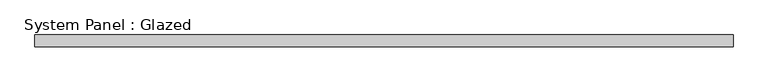
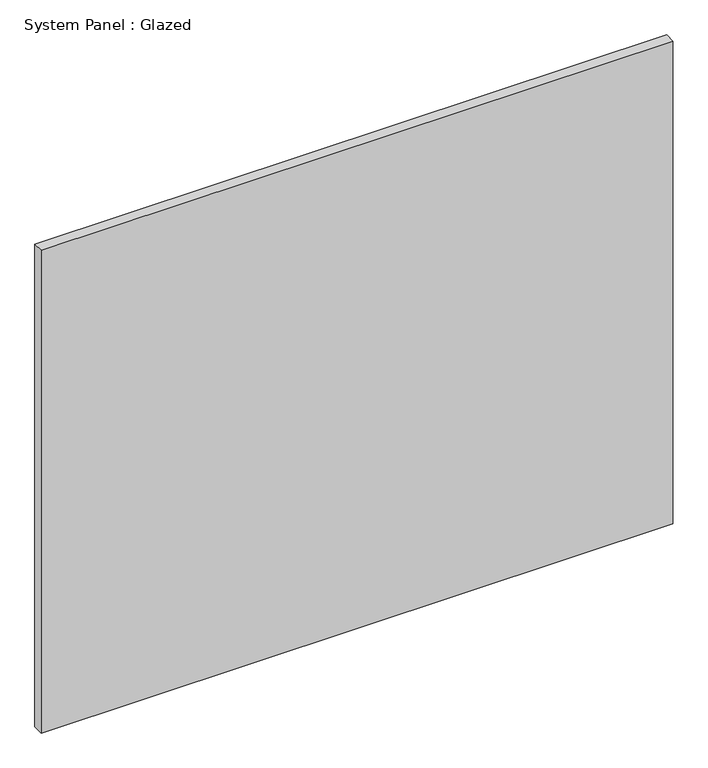
"""IFC4 building model written with IfcOpenShell, lengths in millimetres: plate geometry, System Panel : Glazed."""

import ifcopenshell
import ifcopenshell.guid

model = None  # the IFC model being written
_history = None  # IfcOwnerHistory: only IFC2X3 demands one
_inside = {}  # id of a spatial element -> (the spatial element, [elements in it])
_under = {}  # id of a project, library or spatial element -> (it, [spatial elements below it])
_declared = {}  # id of a project -> (the project, [libraries it declares])
_typed = {}  # id of a type object -> (the type object, [elements of that type])
_made_of = {}  # id of a material, layer set ... -> (it, [elements and type objects made of it])


def new_model(schema):
    """Start an empty IFC model of exactly this schema.

    Asked for "IFC4X3", IfcOpenShell would pick the latest addendum, in which some entities
    have other attributes; the version numbers below select the first issue.
    IFC2X3 requires an IfcOwnerHistory on every rooted entity: one is made here for all.
    """
    global model, _history
    if schema == "IFC4X3":
        model = ifcopenshell.file(schema_version=(4, 3, 0, 0))
    else:
        model = ifcopenshell.file(schema=schema)
    _inside.clear()
    _under.clear()
    _declared.clear()
    _typed.clear()
    _made_of.clear()
    _history = None
    if model.schema == "IFC2X3":
        org = make("IfcOrganization", Name="unknown")
        user = make(
            "IfcPersonAndOrganization",
            ThePerson=make("IfcPerson", FamilyName="unknown"),
            TheOrganization=org,
        )
        app = make(
            "IfcApplication",
            ApplicationDeveloper=org,
            Version="unknown",
            ApplicationFullName="unknown",
            ApplicationIdentifier="unknown",
        )
        _history = make(
            "IfcOwnerHistory",
            OwningUser=user,
            OwningApplication=app,
            ChangeAction="ADDED",
            CreationDate=0,
        )
    return model


def make(cls, **values):
    """One entity of the class cls with the attributes given. An attribute that is None is left unset."""
    return model.create_entity(
        cls, **{name: value for name, value in values.items() if value is not None}
    )


def rooted(cls, **values):
    """An entity with a GlobalId (a new one), such as an element, a storey or a relation."""
    return make(cls, GlobalId=ifcopenshell.guid.new(), OwnerHistory=_history, **values)


def si_unit(unit_type, name, prefix=None):
    """IfcSIUnit, for example si_unit("LENGTHUNIT", "METRE", prefix="MILLI")."""
    return make("IfcSIUnit", UnitType=unit_type, Prefix=prefix, Name=name)


def assignment(units):
    """IfcUnitAssignment: the units of a project."""
    return None if units is None else make("IfcUnitAssignment", Units=units)


def point(xyz):
    """IfcCartesianPoint."""
    return None if xyz is None else make("IfcCartesianPoint", Coordinates=xyz)


def direction(xyz):
    """IfcDirection."""
    return None if xyz is None else make("IfcDirection", DirectionRatios=xyz)


def frame(location, z_axis=None, x_axis=None):
    """IfcAxis2Placement3D, a coordinate frame: its origin and axes. An axis left out is left unset."""
    return make(
        "IfcAxis2Placement3D",
        Location=point(location),
        Axis=direction(z_axis),
        RefDirection=direction(x_axis),
    )


def origin():
    """The frame at (0, 0, 0) with its axes left unset."""
    return frame((0.0, 0.0, 0.0))


def origin_with_axes():
    """The frame at (0, 0, 0) with the z axis (0, 0, 1) and the x axis (1, 0, 0) written out."""
    return frame((0.0, 0.0, 0.0), z_axis=(0.0, 0.0, 1.0), x_axis=(1.0, 0.0, 0.0))


def place(relative_to, where):
    """IfcLocalPlacement: puts the frame where relative to a parent placement (None: the world)."""
    return make(
        "IfcLocalPlacement", PlacementRelTo=relative_to, RelativePlacement=where
    )


def context(
    kind, dimensions, precision=None, world=None, true_north=None, identifier=None
):
    """IfcGeometricRepresentationContext, for example the 3D "Model" context."""
    return make(
        "IfcGeometricRepresentationContext",
        ContextIdentifier=identifier,
        ContextType=kind,
        CoordinateSpaceDimension=dimensions,
        Precision=precision,
        WorldCoordinateSystem=world,
        TrueNorth=true_north,
    )


def project(units=None, contexts=None):
    """IfcProject with its units and contexts."""
    return rooted(
        "IfcProject",
        Name="project",
        RepresentationContexts=contexts,
        UnitsInContext=assignment(units),
    )


def spatial(cls, under=None, at=None, **own):
    """A site, building, storey or space (cls), placed at a placement, below another one or the project."""
    s = rooted(cls, ObjectPlacement=at, **own)
    if under is not None:
        _under.setdefault(under.id(), (under, []))[1].append(s)
    return s


def polyline(points):
    """IfcPolyline through the points."""
    return make("IfcPolyline", Points=[point(p) for p in points])


def outline(outer, holes=None, kind="AREA"):
    """IfcArbitraryClosedProfileDef: a profile drawn as a closed curve; with holes, ...WithVoids."""
    if holes is None:
        return make("IfcArbitraryClosedProfileDef", ProfileType=kind, OuterCurve=outer)
    return make(
        "IfcArbitraryProfileDefWithVoids",
        ProfileType=kind,
        OuterCurve=outer,
        InnerCurves=holes,
    )


def extrude(swept, where, along, depth):
    """IfcExtrudedAreaSolid: the profile swept, set in the frame where, extruded along a direction by depth."""
    return make(
        "IfcExtrudedAreaSolid",
        SweptArea=swept,
        Position=where,
        ExtrudedDirection=direction(along),
        Depth=depth,
    )


def shape(context_of_items, identifier, shape_type, items):
    """IfcShapeRepresentation: the items that make up one representation, for example the "Body"."""
    return make(
        "IfcShapeRepresentation",
        ContextOfItems=context_of_items,
        RepresentationIdentifier=identifier,
        RepresentationType=shape_type,
        Items=items,
    )


def source(mapping_origin, context_of_items, identifier, shape_type, items):
    """IfcRepresentationMap: a shape defined once, which mapped items show again and again."""
    return make(
        "IfcRepresentationMap",
        MappingOrigin=mapping_origin,
        MappedRepresentation=shape(context_of_items, identifier, shape_type, items),
    )


def transform(
    local_origin,
    x_axis=None,
    y_axis=None,
    z_axis=None,
    scale=None,
    scale2=None,
    scale3=None,
    uniform=True,
):
    """IfcCartesianTransformationOperator3D, or its non-uniform kind. x_axis, y_axis, z_axis: its Axis1, 2, 3."""
    if uniform:
        return make(
            "IfcCartesianTransformationOperator3D",
            Axis1=direction(x_axis),
            Axis2=direction(y_axis),
            LocalOrigin=point(local_origin),
            Scale=scale,
            Axis3=direction(z_axis),
        )
    return make(
        "IfcCartesianTransformationOperator3DnonUniform",
        Axis1=direction(x_axis),
        Axis2=direction(y_axis),
        LocalOrigin=point(local_origin),
        Scale=scale,
        Axis3=direction(z_axis),
        Scale2=scale2,
        Scale3=scale3,
    )


def mapped(mapping_source, mapping_target):
    """IfcMappedItem: shows the shape of a source again, moved by a transform."""
    return make(
        "IfcMappedItem", MappingSource=mapping_source, MappingTarget=mapping_target
    )


def made_of(thing, what):
    """Note that an element or type object is made of a material, layer set ...; save() writes the relation."""
    if what is not None:
        _made_of.setdefault(what.id(), (what, []))[1].append(thing)
    return thing


def element(
    cls,
    number,
    at=None,
    inside=None,
    cuts=None,
    type_object=None,
    material=None,
    context=None,
    identifier="Body",
    shape_type=None,
    held_by="IfcProductDefinitionShape",
    body=None,
    shapes=None,
    **own,
):
    """One element of the class cls, such as IfcWall. Its Tag is "e" and its number.

    at: its placement. inside: the storey or other place that contains it. cuts: it is an
    opening in that element (IfcRelVoidsElement). A single representation is given by context,
    identifier, shape_type and body (its items); several are given by shapes. held_by: the class
    of the entity that holds the representations. save() writes the other relations.
    """
    e = rooted(cls, Tag="e%d" % number, ObjectPlacement=at, **own)
    if body is not None:
        shapes = [shape(context, identifier, shape_type, body)]
    if shapes is not None:
        e.Representation = make(held_by, Representations=shapes)
    if inside is not None:
        _inside.setdefault(inside.id(), (inside, []))[1].append(e)
    if cuts is not None:
        rooted(
            "IfcRelVoidsElement", RelatingBuildingElement=cuts, RelatedOpeningElement=e
        )
    if type_object is not None:
        _typed.setdefault(type_object.id(), (type_object, []))[1].append(e)
    return made_of(e, material)


def aggregate(whole, parts):
    """IfcRelAggregates: a whole, such as a stair, and the parts it consists of."""
    return rooted("IfcRelAggregates", RelatingObject=whole, RelatedObjects=parts)


def save(model, path):
    """Write the relations noted so far, then the file.

    IfcRelAggregates (storeys below a building ...), IfcRelContainedInSpatialStructure (elements
    in a storey), IfcRelDefinesByType, IfcRelAssociatesMaterial and IfcRelDeclares: one each for
    every whole, place, type object, material and project.
    """
    for whole, parts in _under.values():
        aggregate(whole, parts)
    for where, things in _inside.values():
        rooted(
            "IfcRelContainedInSpatialStructure",
            RelatedElements=things,
            RelatingStructure=where,
        )
    for kind, things in _typed.values():
        rooted("IfcRelDefinesByType", RelatedObjects=things, RelatingType=kind)
    for what, things in _made_of.values():
        rooted("IfcRelAssociatesMaterial", RelatedObjects=things, RelatingMaterial=what)
    for by, libraries in _declared.values():
        rooted("IfcRelDeclares", RelatingContext=by, RelatedDefinitions=libraries)
    model.write(path)


def system_panel_glazed_ea15e787(model_context):
    return source(origin(), model_context, "Body", "SweptSolid", [
        extrude(outline(polyline([(742.2499998, 24.5), (-742.2499998, 24.5), (-742.2499998, 49.5), (742.2499998, 49.5), (742.2499998, 24.5)])), origin_with_axes(), (0.0, 0.0, 1.0), 1200.0),
    ])


if __name__ == "__main__":
    model = new_model("IFC4")
    model_context = context("Model", 3, world=origin())
    ifc_project = project(units=[si_unit("LENGTHUNIT", "METRE", prefix="MILLI")], contexts=[model_context])
    site = spatial("IfcSite", under=ifc_project)
    building = spatial("IfcBuilding", under=site)
    placement = place(None, origin())
    system_panel_glazed_shape = system_panel_glazed_ea15e787(model_context)
    element("IfcPlate", 1, ObjectType="System Panel : Glazed", at=placement, inside=building, context=model_context, shape_type="MappedRepresentation", body=[
        mapped(system_panel_glazed_shape, transform((0.0, 0.0, 0.0), x_axis=(1.0, 0.0, 0.0), y_axis=(0.0, 1.0, 0.0), z_axis=(0.0, 0.0, 1.0))),
    ])
    save(model, "model.ifc")

# Revit data of these elements
# Element 1 (IfcPlate, "System Panel : Glazed")
#   Materials on its faces: "Glass"
# Materials
#   "Glass": class "Glass", colour RGB 218 227 224, transparency 0.85, Description = "Soda Lime Glass", Cost = 0
